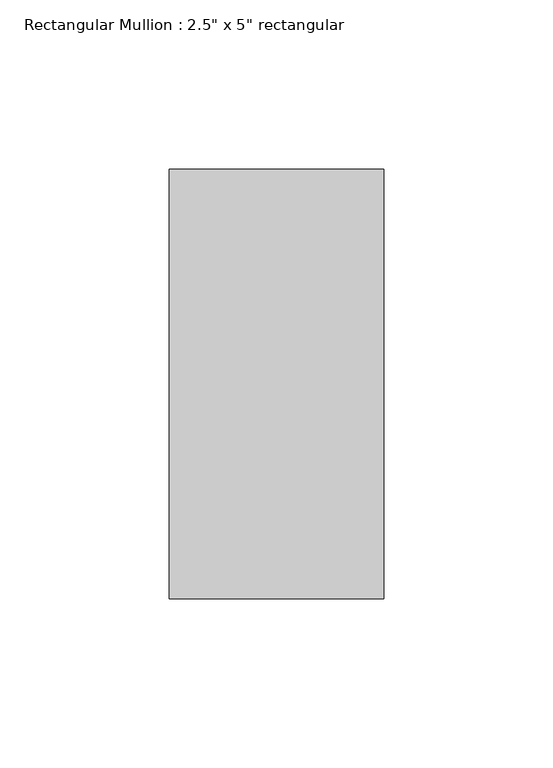
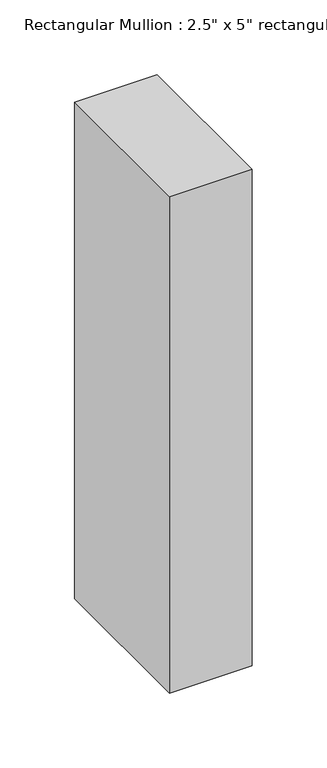
"""IFC4 building model written with IfcOpenShell, lengths in millimetres: member geometry."""

import ifcopenshell
import ifcopenshell.guid

model = None  # the IFC model being written
_history = None  # IfcOwnerHistory: only IFC2X3 demands one
_inside = {}  # id of a spatial element -> (the spatial element, [elements in it])
_under = {}  # id of a project, library or spatial element -> (it, [spatial elements below it])
_declared = {}  # id of a project -> (the project, [libraries it declares])
_typed = {}  # id of a type object -> (the type object, [elements of that type])
_made_of = {}  # id of a material, layer set ... -> (it, [elements and type objects made of it])


def new_model(schema):
    """Start an empty IFC model of exactly this schema.

    Asked for "IFC4X3", IfcOpenShell would pick the latest addendum, in which some entities
    have other attributes; the version numbers below select the first issue.
    IFC2X3 requires an IfcOwnerHistory on every rooted entity: one is made here for all.
    """
    global model, _history
    if schema == "IFC4X3":
        model = ifcopenshell.file(schema_version=(4, 3, 0, 0))
    else:
        model = ifcopenshell.file(schema=schema)
    _inside.clear()
    _under.clear()
    _declared.clear()
    _typed.clear()
    _made_of.clear()
    _history = None
    if model.schema == "IFC2X3":
        org = make("IfcOrganization", Name="unknown")
        user = make(
            "IfcPersonAndOrganization",
            ThePerson=make("IfcPerson", FamilyName="unknown"),
            TheOrganization=org,
        )
        app = make(
            "IfcApplication",
            ApplicationDeveloper=org,
            Version="unknown",
            ApplicationFullName="unknown",
            ApplicationIdentifier="unknown",
        )
        _history = make(
            "IfcOwnerHistory",
            OwningUser=user,
            OwningApplication=app,
            ChangeAction="ADDED",
            CreationDate=0,
        )
    return model


def make(cls, **values):
    """One entity of the class cls with the attributes given. An attribute that is None is left unset."""
    return model.create_entity(
        cls, **{name: value for name, value in values.items() if value is not None}
    )


def rooted(cls, **values):
    """An entity with a GlobalId (a new one), such as an element, a storey or a relation."""
    return make(cls, GlobalId=ifcopenshell.guid.new(), OwnerHistory=_history, **values)


def si_unit(unit_type, name, prefix=None):
    """IfcSIUnit, for example si_unit("LENGTHUNIT", "METRE", prefix="MILLI")."""
    return make("IfcSIUnit", UnitType=unit_type, Prefix=prefix, Name=name)


def assignment(units):
    """IfcUnitAssignment: the units of a project."""
    return None if units is None else make("IfcUnitAssignment", Units=units)


def point(xyz):
    """IfcCartesianPoint."""
    return None if xyz is None else make("IfcCartesianPoint", Coordinates=xyz)


def direction(xyz):
    """IfcDirection."""
    return None if xyz is None else make("IfcDirection", DirectionRatios=xyz)


def frame(location, z_axis=None, x_axis=None):
    """IfcAxis2Placement3D, a coordinate frame: its origin and axes. An axis left out is left unset."""
    return make(
        "IfcAxis2Placement3D",
        Location=point(location),
        Axis=direction(z_axis),
        RefDirection=direction(x_axis),
    )


def origin():
    """The frame at (0, 0, 0) with its axes left unset."""
    return frame((0.0, 0.0, 0.0))


def place(relative_to, where):
    """IfcLocalPlacement: puts the frame where relative to a parent placement (None: the world)."""
    return make(
        "IfcLocalPlacement", PlacementRelTo=relative_to, RelativePlacement=where
    )


def context(
    kind, dimensions, precision=None, world=None, true_north=None, identifier=None
):
    """IfcGeometricRepresentationContext, for example the 3D "Model" context."""
    return make(
        "IfcGeometricRepresentationContext",
        ContextIdentifier=identifier,
        ContextType=kind,
        CoordinateSpaceDimension=dimensions,
        Precision=precision,
        WorldCoordinateSystem=world,
        TrueNorth=true_north,
    )


def project(units=None, contexts=None):
    """IfcProject with its units and contexts."""
    return rooted(
        "IfcProject",
        Name="project",
        RepresentationContexts=contexts,
        UnitsInContext=assignment(units),
    )


def spatial(cls, under=None, at=None, **own):
    """A site, building, storey or space (cls), placed at a placement, below another one or the project."""
    s = rooted(cls, ObjectPlacement=at, **own)
    if under is not None:
        _under.setdefault(under.id(), (under, []))[1].append(s)
    return s


def polyline(points):
    """IfcPolyline through the points."""
    return make("IfcPolyline", Points=[point(p) for p in points])


def outline(outer, holes=None, kind="AREA"):
    """IfcArbitraryClosedProfileDef: a profile drawn as a closed curve; with holes, ...WithVoids."""
    if holes is None:
        return make("IfcArbitraryClosedProfileDef", ProfileType=kind, OuterCurve=outer)
    return make(
        "IfcArbitraryProfileDefWithVoids",
        ProfileType=kind,
        OuterCurve=outer,
        InnerCurves=holes,
    )


def extrude(swept, where, along, depth):
    """IfcExtrudedAreaSolid: the profile swept, set in the frame where, extruded along a direction by depth."""
    return make(
        "IfcExtrudedAreaSolid",
        SweptArea=swept,
        Position=where,
        ExtrudedDirection=direction(along),
        Depth=depth,
    )


def shape(context_of_items, identifier, shape_type, items):
    """IfcShapeRepresentation: the items that make up one representation, for example the "Body"."""
    return make(
        "IfcShapeRepresentation",
        ContextOfItems=context_of_items,
        RepresentationIdentifier=identifier,
        RepresentationType=shape_type,
        Items=items,
    )


def source(mapping_origin, context_of_items, identifier, shape_type, items):
    """IfcRepresentationMap: a shape defined once, which mapped items show again and again."""
    return make(
        "IfcRepresentationMap",
        MappingOrigin=mapping_origin,
        MappedRepresentation=shape(context_of_items, identifier, shape_type, items),
    )


def transform(
    local_origin,
    x_axis=None,
    y_axis=None,
    z_axis=None,
    scale=None,
    scale2=None,
    scale3=None,
    uniform=True,
):
    """IfcCartesianTransformationOperator3D, or its non-uniform kind. x_axis, y_axis, z_axis: its Axis1, 2, 3."""
    if uniform:
        return make(
            "IfcCartesianTransformationOperator3D",
            Axis1=direction(x_axis),
            Axis2=direction(y_axis),
            LocalOrigin=point(local_origin),
            Scale=scale,
            Axis3=direction(z_axis),
        )
    return make(
        "IfcCartesianTransformationOperator3DnonUniform",
        Axis1=direction(x_axis),
        Axis2=direction(y_axis),
        LocalOrigin=point(local_origin),
        Scale=scale,
        Axis3=direction(z_axis),
        Scale2=scale2,
        Scale3=scale3,
    )


def mapped(mapping_source, mapping_target):
    """IfcMappedItem: shows the shape of a source again, moved by a transform."""
    return make(
        "IfcMappedItem", MappingSource=mapping_source, MappingTarget=mapping_target
    )


def made_of(thing, what):
    """Note that an element or type object is made of a material, layer set ...; save() writes the relation."""
    if what is not None:
        _made_of.setdefault(what.id(), (what, []))[1].append(thing)
    return thing


def element(
    cls,
    number,
    at=None,
    inside=None,
    cuts=None,
    type_object=None,
    material=None,
    context=None,
    identifier="Body",
    shape_type=None,
    held_by="IfcProductDefinitionShape",
    body=None,
    shapes=None,
    **own,
):
    """One element of the class cls, such as IfcWall. Its Tag is "e" and its number.

    at: its placement. inside: the storey or other place that contains it. cuts: it is an
    opening in that element (IfcRelVoidsElement). A single representation is given by context,
    identifier, shape_type and body (its items); several are given by shapes. held_by: the class
    of the entity that holds the representations. save() writes the other relations.
    """
    e = rooted(cls, Tag="e%d" % number, ObjectPlacement=at, **own)
    if body is not None:
        shapes = [shape(context, identifier, shape_type, body)]
    if shapes is not None:
        e.Representation = make(held_by, Representations=shapes)
    if inside is not None:
        _inside.setdefault(inside.id(), (inside, []))[1].append(e)
    if cuts is not None:
        rooted(
            "IfcRelVoidsElement", RelatingBuildingElement=cuts, RelatedOpeningElement=e
        )
    if type_object is not None:
        _typed.setdefault(type_object.id(), (type_object, []))[1].append(e)
    return made_of(e, material)


def aggregate(whole, parts):
    """IfcRelAggregates: a whole, such as a stair, and the parts it consists of."""
    return rooted("IfcRelAggregates", RelatingObject=whole, RelatedObjects=parts)


def save(model, path):
    """Write the relations noted so far, then the file.

    IfcRelAggregates (storeys below a building ...), IfcRelContainedInSpatialStructure (elements
    in a storey), IfcRelDefinesByType, IfcRelAssociatesMaterial and IfcRelDeclares: one each for
    every whole, place, type object, material and project.
    """
    for whole, parts in _under.values():
        aggregate(whole, parts)
    for where, things in _inside.values():
        rooted(
            "IfcRelContainedInSpatialStructure",
            RelatedElements=things,
            RelatingStructure=where,
        )
    for kind, things in _typed.values():
        rooted("IfcRelDefinesByType", RelatedObjects=things, RelatingType=kind)
    for what, things in _made_of.values():
        rooted("IfcRelAssociatesMaterial", RelatedObjects=things, RelatingMaterial=what)
    for by, libraries in _declared.values():
        rooted("IfcRelDeclares", RelatingContext=by, RelatedDefinitions=libraries)
    model.write(path)


def member_2d477cc6(model_context):
    return source(origin(), model_context, "Body", "SweptSolid", [
        extrude(outline(polyline([(31.75, 63.5), (31.75, -63.5), (-31.75, -63.5), (-31.75, 63.5), (31.75, 63.5)])), frame((0.0, 0.0, -404.75), z_axis=(0.0, 0.0, 1.0), x_axis=(1.0, 0.0, 0.0)), (0.0, 0.0, 1.0), 404.75),
    ])


if __name__ == "__main__":
    model = new_model("IFC4")
    model_context = context("Model", 3, world=origin())
    ifc_project = project(units=[si_unit("LENGTHUNIT", "METRE", prefix="MILLI")], contexts=[model_context])
    site = spatial("IfcSite", under=ifc_project)
    building = spatial("IfcBuilding", under=site)
    placement = place(None, origin())
    member_shape = member_2d477cc6(model_context)
    element("IfcMember", 1, ObjectType="Rectangular Mullion : 2.5\" x 5\" rectangular", at=placement, inside=building, context=model_context, shape_type="MappedRepresentation", body=[
        mapped(member_shape, transform((0.0, 0.0, 0.0), x_axis=(1.0, 0.0, 0.0), y_axis=(0.0, 1.0, 0.0), z_axis=(0.0, 0.0, 1.0))),
    ])
    save(model, "model.ifc")

# Revit data of these elements
# Type "Rectangular Mullion : 2.5\" x 5\" rectangular"
#   built-in parameter 1007304 = 0.416667 (stored number, unit not read)
#   built-in parameter 1007301 = 0.104167 (stored number, unit not read)
#   built-in parameter 1007300 = 0.104167 (stored number, unit not read)
# Element 1 (IfcMember, "Rectangular Mullion : 2.5\" x 5\" rectangular")
#   Materials on its faces: "Metal - Aluminum 2"
# Materials
#   "Metal - Aluminum 2": class "Metal", colour RGB 189 187 185, transparency 0
